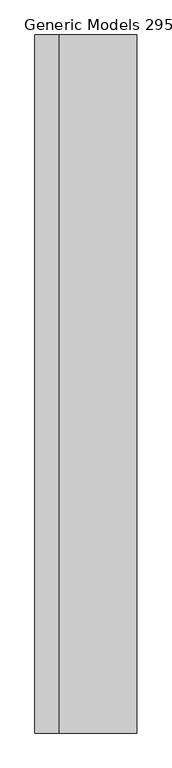
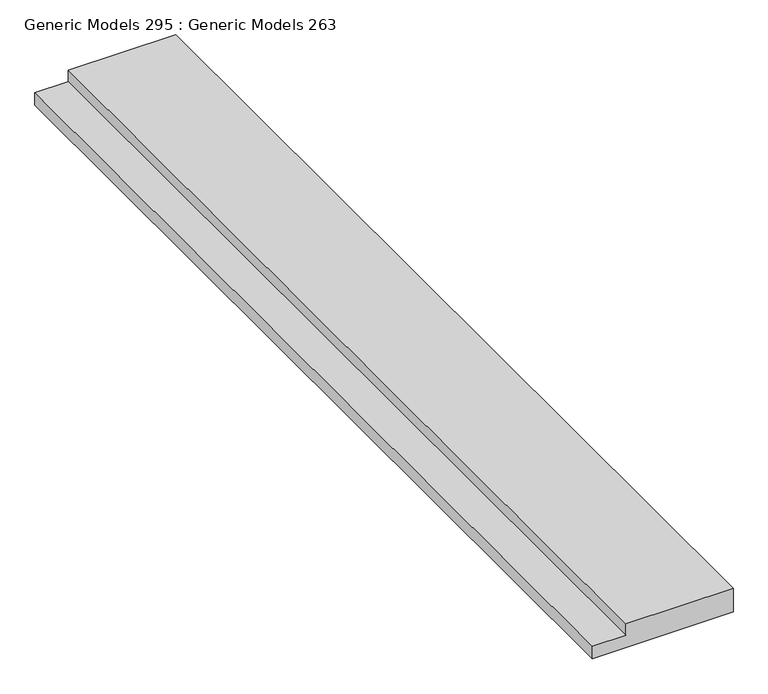
"""IFC4 building model written with IfcOpenShell, lengths in millimetres: proxy geometry, Generic Models 295 : Generic Models 263."""

from ifc_helpers import new_model, si_unit, frame, origin, place, context, project, spatial, polyline, outline, extrude, source, transform, mapped, element, save


def generic_models_295_generic_models_263_197a9b76(model_context):
    return source(origin(), model_context, "Body", "SweptSolid", [
        extrude(outline(polyline([(-381.0, 92037.1797726), (-381.0, 91579.9797726), (-558.8, 91579.9797726), (-558.8, 93498.3966125), (-215.9, 93498.3966125), (-215.9, 92037.1797726), (-381.0, 92037.1797726)])), frame((0.0, -4692.2809088, 0.0), z_axis=(0.0, 1.0, 0.0), x_axis=(0.0, 0.0, 1.0)), (0.0, 0.0, 1.0), 13158.0645094),
    ])


if __name__ == "__main__":
    model = new_model("IFC4")
    model_context = context("Model", 3, world=origin())
    ifc_project = project(units=[si_unit("LENGTHUNIT", "METRE", prefix="MILLI")], contexts=[model_context])
    site = spatial("IfcSite", under=ifc_project)
    building = spatial("IfcBuilding", under=site)
    placement = place(None, origin())
    generic_models_295_generic_models_263_shape = generic_models_295_generic_models_263_197a9b76(model_context)
    element("IfcBuildingElementProxy", 1, Name="Generic Models 295 : Generic Models 263", ObjectType="Generic Models 295 : Generic Models 263", at=placement, inside=building, context=model_context, shape_type="MappedRepresentation", body=[
        mapped(generic_models_295_generic_models_263_shape, transform((0.0, 0.0, 0.0), x_axis=(1.0, 0.0, 0.0), y_axis=(0.0, 1.0, 0.0), z_axis=(0.0, 0.0, 1.0))),
    ])
    save(model, "model.ifc")

# Revit data of these elements
# Element 1 (IfcBuildingElementProxy, "Generic Models 295 : Generic Models 263")
#   Materials on its faces: "CRUSHED AGGREGATE BASE COURSE"
# Materials
#   "CRUSHED AGGREGATE BASE COURSE": class "Miscellaneous", colour RGB 183 184 198, transparency 0, Cost = 0
